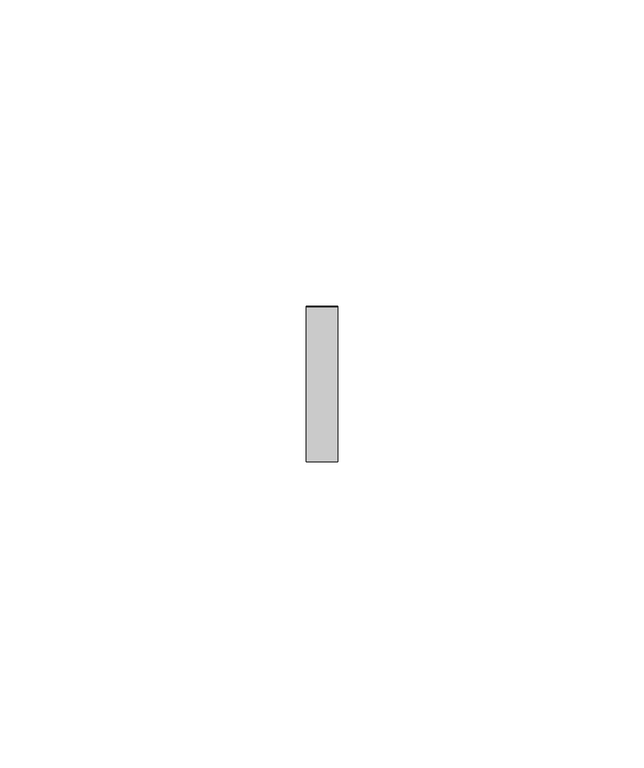
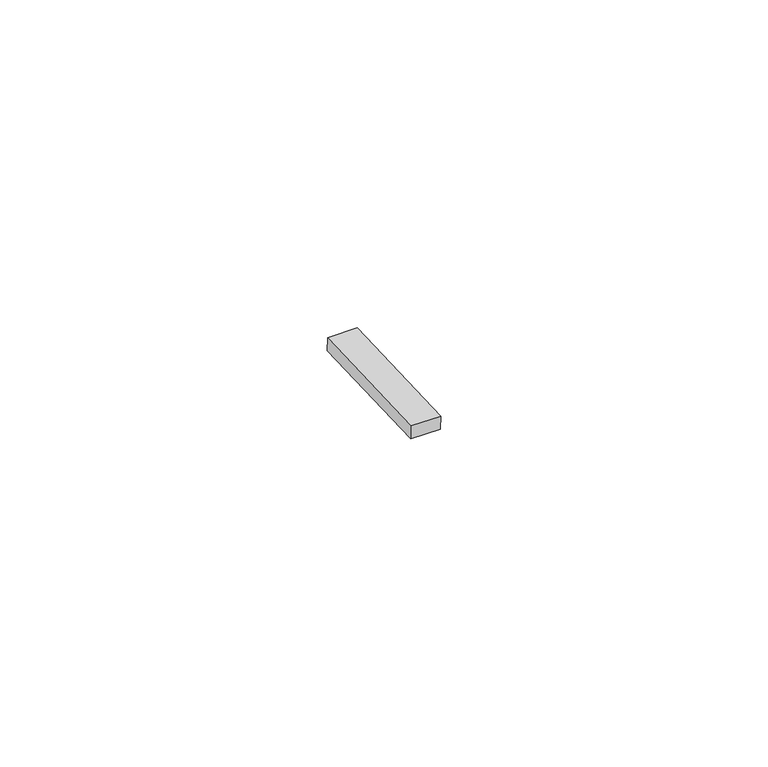
"""IFC4 building model written with IfcOpenShell, lengths in millimetres: proxy geometry, Inner panel:Inner panel:1:Inner panel:1 : Inner panel:Inner panel:300324:2:Inner panel:1:Inner panel:1 : Inner panel:Inner panel:300324:2 : Inner panel:Inner panel:1:Inner panel:1 : Inner panel:Inner panel:300324:300043:109 : Inner panel:Inner panel:1:Inner panel:1 : Inner panel:Inner panel:300324:2:Inner panel:1:Inner panel:1 : Inner panel:Inner panel:300324:2 : Inner panel:Inner panel:1:Inner panel:1 : Inner panel:Inner panel:300324:300043:308120."""

from ifc_helpers import new_model, si_unit, frame, origin, place, context, project, spatial, polyline, outline, extrude, source, transform, mapped, element, save


def generic_models_ceedae5a(model_context):
    return source(origin(), model_context, "Body", "SweptSolid", [
        extrude(outline(polyline([(0.0, -25.3999999), (0.0, 0.0), (5.2138089, 0.0), (5.2138089, -25.3999999), (0.0, -25.3999999)])), frame((593530.195117, -578962.7476805, 3951.4793391), z_axis=(0.0, -0.041630544712223896, 0.9991330730923502), x_axis=(-1.0, 0.0, 0.0)), (0.0, 0.0, 1.0), 2.4763745),
    ])


if __name__ == "__main__":
    model = new_model("IFC4")
    model_context = context("Model", 3, world=origin())
    ifc_project = project(units=[si_unit("LENGTHUNIT", "METRE", prefix="MILLI")], contexts=[model_context])
    site = spatial("IfcSite", under=ifc_project)
    building = spatial("IfcBuilding", under=site)
    placement = place(None, origin())
    generic_models_shape = generic_models_ceedae5a(model_context)
    element("IfcBuildingElementProxy", 1, Name="Inner panel:Inner panel:1:Inner panel:1 : Inner panel:Inner panel:300324:2:Inner panel:1:Inner panel:1 : Inner panel:Inner panel:300324:2 : Inner panel:Inner panel:1:Inner panel:1 : Inner panel:Inner panel:300324:300043:109 : Inner panel:Inner panel:1:Inner panel:1 : Inner panel:Inner panel:300324:2:Inner panel:1:Inner panel:1 : Inner panel:Inner panel:300324:2 : Inner panel:Inner panel:1:Inner panel:1 : Inner panel:Inner panel:300324:300043:308120", ObjectType="Inner panel:Inner panel:1:Inner panel:1 : Inner panel:Inner panel:300324:2:Inner panel:1:Inner panel:1 : Inner panel:Inner panel:300324:2 : Inner panel:Inner panel:1:Inner panel:1 : Inner panel:Inner panel:300324:300043:109 : Inner panel:Inner panel:1:Inner panel:1 : Inner panel:Inner panel:300324:2:Inner panel:1:Inner panel:1 : Inner panel:Inner panel:300324:2 : Inner panel:Inner panel:1:Inner panel:1 : Inner panel:Inner panel:300324:300043:308120", at=placement, inside=building, context=model_context, shape_type="MappedRepresentation", body=[
        mapped(generic_models_shape, transform((0.0, 0.0, 0.0), x_axis=(1.0, 0.0, 0.0), y_axis=(0.0, 1.0, 0.0), z_axis=(0.0, 0.0, 1.0))),
    ])
    save(model, "model.ifc")

# Revit data of these elements
# Type "Inner panel:Inner panel:1:Inner panel:1 : Inner panel:Inner panel:300324:2:Inner panel:1:Inner panel:1 : Inner panel:Inner panel:300324:2 : Inner panel:Inner panel:1:Inner panel:1 : Inner panel:Inner panel:300324:300043:109 : Inner panel:Inner panel:1:Inner panel:1 : Inner panel:Inner panel:300324:2:Inner panel:1:Inner panel:1 : Inner panel:Inner panel:300324:2 : Inner panel:Inner panel:1:Inner panel:1 : Inner panel:Inner panel:300324:300043:308120"
#   NameOverride = "Inner panel:Inner panel:1:Inner panel:1 : Inner panel:Inner panel:300324:2:Inner panel:1:Inner panel:1 : Inner panel:Inner panel:300324:2 : Inner panel:Inner panel:1:Inner panel:1 : Inner panel:Inner panel:300324:300043:308120"
#   ObjectTypeOverride = "Inner panel:1:Inner panel:1 : Inner panel:Inner panel:300324:2 : Inner panel:Inner panel:1:Inner panel:1 : Inner panel:Inner panel:300324:300043"
#   Reference = "Inner panel"
#   Tag = "308120"
# Element 1 (IfcBuildingElementProxy, "Inner panel:Inner panel:1:Inner panel:1 : Inner panel:Inner panel:300324:2:Inner panel:1:Inner panel:1 : Inner panel:Inner panel:300324:2 : Inner panel:Inner panel:1:Inner panel:1 : Inner panel:Inner panel:300324:300043:109 : Inner panel:Inner panel:1:Inner panel:1 : Inner panel:Inner panel:300324:2:Inner panel:1:Inner panel:1 : Inner panel:Inner panel:300324:2 : Inner panel:Inner panel:1:Inner panel:1 : Inner panel:Inner panel:300324:300043:308120")
#   Materials on its faces: "AT CLIP - 1\" WIDE NON ABSORBENT, WEATHER-RESISTANT NEOPRENE/EPDM/SBR FOAM"
# Materials
#   "AT CLIP - 1\" WIDE NON ABSORBENT, WEATHER-RESISTANT NEOPRENE/EPDM/SBR FOAM": class "Generic", colour RGB 85 85 85, transparency 0, Cost = 0
